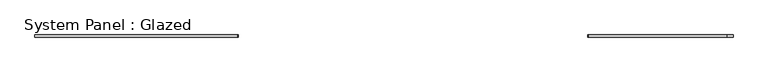
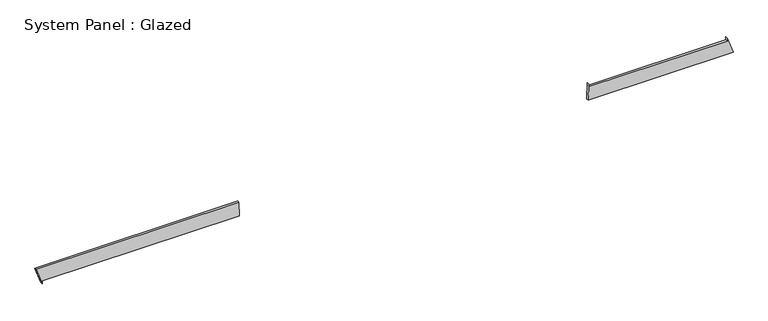
"""IFC4 building model written with IfcOpenShell, lengths in millimetres: plate geometry, System Panel : Glazed."""

from ifc_helpers import new_model, si_unit, frame, origin, place, context, project, spatial, polyline, outline, extrude, source, transform, mapped, element, save


def system_panel_glazed_8560ee69(model_context):
    return source(origin(), model_context, "Body", "SweptSolid", [
        extrude(outline(polyline([(0.0, -3957.3100251), (35.3553391, -3957.3100251), (35.3553391, -1681.6472536), (199.0311077, -1684.9000765), (198.9981604, -4026.9402223), (0.0, -3957.3100251)])), frame((0.0, -49.5, 0.0), z_axis=(0.0, 1.0, 0.0), x_axis=(0.0, 0.0, 1.0)), (0.0, 0.0, 1.0), 25.0),
        extrude(outline(polyline([(35.3553391, 2351.2150268), (35.3553391, 4026.9402223), (234.465824, 3957.5777852), (199.110485, 3957.5782826), (199.0879655, 2356.7975845), (234.4433046, 2356.7970871), (35.3553391, 2351.2150268)])), frame((0.0, -49.5, 0.0), z_axis=(0.0, 1.0, 0.0), x_axis=(0.0, 0.0, 1.0)), (0.0, 0.0, 1.0), 25.0),
    ])


if __name__ == "__main__":
    model = new_model("IFC4")
    model_context = context("Model", 3, world=origin())
    ifc_project = project(units=[si_unit("LENGTHUNIT", "METRE", prefix="MILLI")], contexts=[model_context])
    site = spatial("IfcSite", under=ifc_project)
    building = spatial("IfcBuilding", under=site)
    placement = place(None, origin())
    system_panel_glazed_shape = system_panel_glazed_8560ee69(model_context)
    element("IfcPlate", 1, ObjectType="System Panel : Glazed", at=placement, inside=building, context=model_context, shape_type="MappedRepresentation", body=[
        mapped(system_panel_glazed_shape, transform((0.0, 0.0, 0.0), x_axis=(1.0, 0.0, 0.0), y_axis=(0.0, 1.0, 0.0), z_axis=(0.0, 0.0, 1.0))),
    ])
    save(model, "model.ifc")

# Revit data of these elements
# Element 1 (IfcPlate, "System Panel : Glazed")
#   Materials on its faces: "Glass"
# Materials
#   "Glass": class "Glass", colour RGB 218 227 224, transparency 0.85, Description = "Soda Lime Glass", Cost = 0
